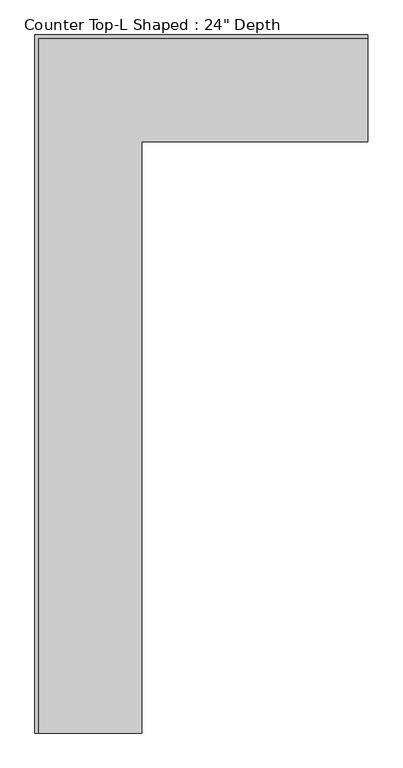
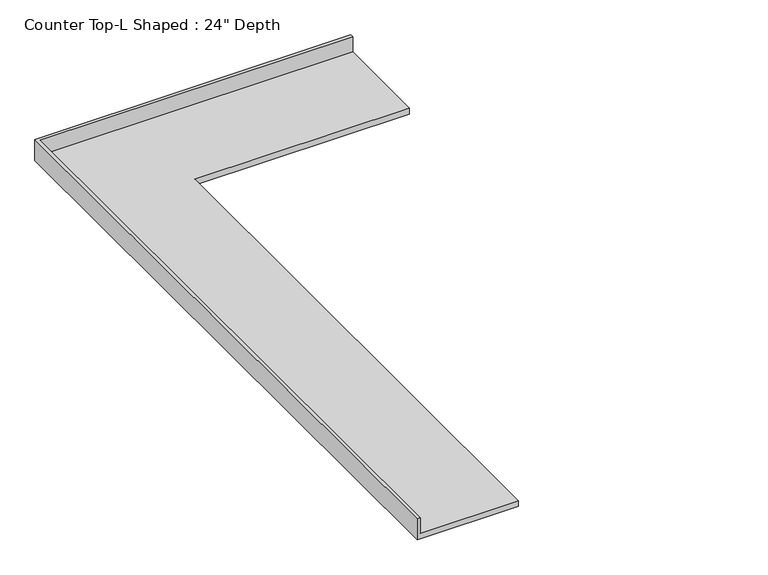
"""IFC4 building model written with IfcOpenShell, lengths in millimetres: furniture geometry."""

from ifc_helpers import new_model, si_unit, origin, place, context, project, spatial, faceted_brep, source, transform, mapped, element, save


def furniture_af42006d(model_context):
    return source(origin(), model_context, "Body", "Brep", [
        faceted_brep([(-565.4622951, -4152.9, 914.4), (-565.4622951, -635.0, 914.4), (780.7377049, -635.0, 914.4), (780.7377049, -19.05, 914.4), (-1181.4122951, -19.05, 914.4), (-1181.4122951, -4152.9, 914.4), (780.7377049, 0.0, 876.3), (780.7377049, -635.0, 876.3), (-565.4622951, -635.0, 876.3), (-565.4622951, -4152.9, 876.3), (-1200.4622951, -4152.9, 876.3), (-1200.4622951, 0.0, 876.3), (-1200.4622951, 0.0, 1016.0), (780.7377049, 0.0, 1016.0), (-1200.4622951, -4152.9, 1016.0), (-1181.4122951, -4152.9, 1016.0), (780.7377049, -19.05, 1016.0), (-1181.4122951, -19.05, 1016.0)], [[[0, 1, 2, 3, 4, 5]], [[6, 7, 8, 9, 10, 11]], [[6, 11, 12, 13]], [[11, 10, 14, 12]], [[14, 10, 9, 0, 5, 15]], [[1, 0, 9, 8]], [[2, 1, 8, 7]], [[7, 6, 13, 16, 3, 2]], [[12, 14, 15, 17, 16, 13]], [[3, 16, 17, 4]], [[17, 15, 5, 4]]]),
    ])


if __name__ == "__main__":
    model = new_model("IFC4")
    model_context = context("Model", 3, world=origin())
    ifc_project = project(units=[si_unit("LENGTHUNIT", "METRE", prefix="MILLI")], contexts=[model_context])
    site = spatial("IfcSite", under=ifc_project)
    building = spatial("IfcBuilding", under=site)
    placement = place(None, origin())
    furniture_shape = furniture_af42006d(model_context)
    element("IfcFurniture", 1, ObjectType="Counter Top-L Shaped : 24\" Depth", at=placement, inside=building, context=model_context, shape_type="MappedRepresentation", body=[
        mapped(furniture_shape, transform((0.0, 0.0, 0.0), x_axis=(1.0, 0.0, 0.0), y_axis=(0.0, 1.0, 0.0), z_axis=(0.0, 0.0, 1.0))),
    ])
    save(model, "model.ifc")

# Revit data of these elements
# Type "Counter Top-L Shaped : 24\" Depth"
#   Assembly Code = "C1030400"
#   Counter Thickness = 0' - 1 1/2"
#   Depth = 2' - 1"
#   Height = 3' - 0"
#   Length - Leg 1 [instance default] = 8' - 0"
#   Length - Leg 2 [instance default] = 6' - 0"
#   Counter Top Material = none
#   Default Elevation = 0
# Element 1 (IfcFurniture, "Counter Top-L Shaped : 24\" Depth")
#   Length - Leg 1 = 6' - 6"
#   Length - Leg 2 = 13' - 7 1/2"
#   Materials on its faces: "Counter Top"
# Materials
#   "Counter Top": class "Wood", colour RGB 226 177 128, transparency 0
